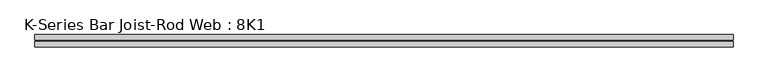
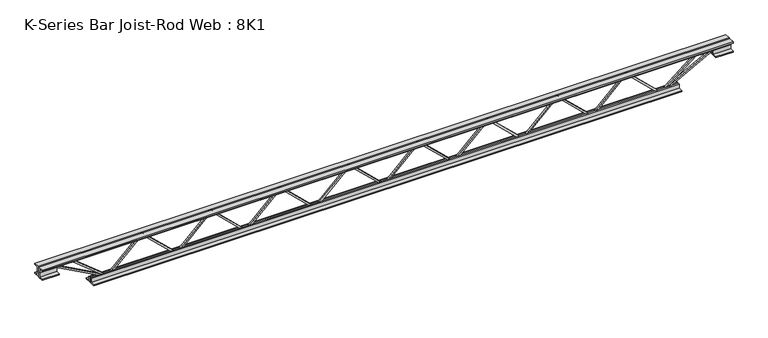
"""IFC4 building model written with IfcOpenShell, lengths in millimetres: beam geometry, K-Series Bar Joist-Rod Web : 8K1."""

from ifc_helpers import new_model, si_unit, frame, origin, place, context, project, spatial, polyline, outline, extrude, source, transform, mapped, element, save


def k_series_bar_joist_rod_web_8k1_28d6b3e6(model_context):
    return source(origin(), model_context, "Body", "SweptSolid", [
        extrude(outline(polyline([(-90.4875, 818.071879), (-100.0125, 818.071879), (-100.0125, 823.1647607), (90.4875, 1021.3327305), (90.4875, 1023.8469671), (-100.0125, 1222.0149368), (-100.0125, 1227.1078185), (-90.4875, 1227.1078185), (-90.4875, 1225.8507002), (100.0125, 1027.6827305), (100.0125, 1017.4969671), (-90.4875, 819.3289973), (-90.4875, 818.071879)])), frame((0.0, -4.7625, 0.0), z_axis=(0.0, 1.0, 0.0), x_axis=(0.0, 0.0, 1.0)), (0.0, 0.0, 1.0), 9.525),
        extrude(outline(polyline([(-90.4875, 409.0359395), (-100.0125, 409.0359395), (-100.0125, 414.1288212), (90.4875, 612.296791), (90.4875, 614.8110276), (-100.0125, 812.9789973), (-100.0125, 818.071879), (-90.4875, 818.071879), (-90.4875, 816.8147607), (100.0125, 618.646791), (100.0125, 608.4610276), (-90.4875, 410.2930578), (-90.4875, 409.0359395)])), frame((0.0, -4.7625, 0.0), z_axis=(0.0, 1.0, 0.0), x_axis=(0.0, 0.0, 1.0)), (0.0, 0.0, 1.0), 9.525),
        extrude(outline(polyline([(-90.4875, 0.0), (-100.0125, 0.0), (-100.0125, 5.0928817), (90.4875, 203.2608514), (90.4875, 205.7750881), (-100.0125, 403.9430578), (-100.0125, 409.0359395), (-90.4875, 409.0359395), (-90.4875, 407.7788212), (100.0125, 209.6108514), (100.0125, 199.4250881), (-90.4875, 1.2571183), (-90.4875, 0.0)])), frame((0.0, -4.7625, 0.0), z_axis=(0.0, 1.0, 0.0), x_axis=(0.0, 0.0, 1.0)), (0.0, 0.0, 1.0), 9.525),
        extrude(outline(polyline([(-90.4875, -409.0359395), (-100.0125, -409.0359395), (-100.0125, -403.9430578), (90.4875, -205.7750881), (90.4875, -203.2608514), (-100.0125, -5.0928817), (-100.0125, 0.0), (-90.4875, 0.0), (-90.4875, -1.2571183), (100.0125, -199.4250881), (100.0125, -209.6108514), (-90.4875, -407.7788212), (-90.4875, -409.0359395)])), frame((0.0, -4.7625, 0.0), z_axis=(0.0, 1.0, 0.0), x_axis=(0.0, 0.0, 1.0)), (0.0, 0.0, 1.0), 9.525),
        extrude(outline(polyline([(-90.4875, -818.071879), (-100.0125, -818.071879), (-100.0125, -812.9789973), (90.4875, -614.8110276), (90.4875, -612.296791), (-100.0125, -414.1288212), (-100.0125, -409.0359395), (-90.4875, -409.0359395), (-90.4875, -410.2930578), (100.0125, -608.4610276), (100.0125, -618.646791), (-90.4875, -816.8147607), (-90.4875, -818.071879)])), frame((0.0, -4.7625, 0.0), z_axis=(0.0, 1.0, 0.0), x_axis=(0.0, 0.0, 1.0)), (0.0, 0.0, 1.0), 9.525),
        extrude(outline(polyline([(-90.4875, -1227.1078185), (-100.0125, -1227.1078185), (-100.0125, -1222.0149368), (90.4875, -1023.8469671), (90.4875, -1021.3327305), (-100.0125, -823.1647607), (-100.0125, -818.071879), (-90.4875, -818.071879), (-90.4875, -819.3289973), (100.0125, -1017.4969671), (100.0125, -1027.6827305), (-90.4875, -1225.8507002), (-90.4875, -1227.1078185)])), frame((0.0, -4.7625, 0.0), z_axis=(0.0, 1.0, 0.0), x_axis=(0.0, 0.0, 1.0)), (0.0, 0.0, 1.0), 9.525),
        extrude(outline(polyline([(-90.4875, 1227.1078185), (-100.0125, 1227.1078185), (-100.0125, 1232.2007002), (90.4875, 1430.36867), (90.4875, 1432.8829066), (-100.0125, 1631.0508764), (-100.0125, 1636.143758), (-90.4875, 1636.143758), (-90.4875, 1634.8866397), (100.0125, 1436.71867), (100.0125, 1426.5329066), (-90.4875, 1228.3649368), (-90.4875, 1227.1078185)])), frame((0.0, -4.7625, 0.0), z_axis=(0.0, 1.0, 0.0), x_axis=(0.0, 0.0, 1.0)), (0.0, 0.0, 1.0), 9.525),
        extrude(outline(polyline([(-90.4875, -1636.143758), (-100.0125, -1636.143758), (-100.0125, -1631.0508764), (90.4875, -1432.8829066), (90.4875, -1430.36867), (-100.0125, -1232.2007002), (-100.0125, -1227.1078185), (-90.4875, -1227.1078185), (-90.4875, -1228.3649368), (100.0125, -1426.5329066), (100.0125, -1436.71867), (-90.4875, -1634.8866397), (-90.4875, -1636.143758)])), frame((0.0, -4.7625, 0.0), z_axis=(0.0, 1.0, 0.0), x_axis=(0.0, 0.0, 1.0)), (0.0, 0.0, 1.0), 9.525),
        extrude(outline(polyline([(4.7625, 101.6), (36.5125, 101.6), (36.5125, 95.25), (11.1125, 95.25), (11.1125, 69.85), (4.7625, 69.85), (4.7625, 101.6)])), frame((-2042.543758, 0.0, 0.0), z_axis=(1.0, 0.0, 0.0), x_axis=(0.0, 1.0, 0.0)), (0.0, 0.0, 1.0), 4085.0875161),
        extrude(outline(polyline([(-4.7625, 101.6), (-4.7625, 69.85), (-11.1125, 69.85), (-11.1125, 95.25), (-36.5125, 95.25), (-36.5125, 101.6), (-4.7625, 101.6)])), frame((-2042.543758, 0.0, 0.0), z_axis=(1.0, 0.0, 0.0), x_axis=(0.0, 1.0, 0.0)), (0.0, 0.0, 1.0), 4085.0875161),
        extrude(outline(polyline([(-4.7625, 38.1), (-36.5125, 38.1), (-36.5125, 44.45), (-11.1125, 44.45), (-11.1125, 69.85), (-4.7625, 69.85), (-4.7625, 38.1)])), frame((-2042.543758, 0.0, 0.0), z_axis=(1.0, 0.0, 0.0), x_axis=(0.0, 1.0, 0.0)), (0.0, 0.0, 1.0), 101.6),
        extrude(outline(polyline([(36.5125, 38.1), (4.7625, 38.1), (4.7625, 69.85), (11.1125, 69.85), (11.1125, 44.45), (36.5125, 44.45), (36.5125, 38.1)])), frame((-2042.543758, 0.0, 0.0), z_axis=(1.0, 0.0, 0.0), x_axis=(0.0, 1.0, 0.0)), (0.0, 0.0, 1.0), 101.6),
        extrude(outline(polyline([(4.7625, 38.1), (4.7625, 69.85), (11.1125, 69.85), (11.1125, 44.45), (36.5125, 44.45), (36.5125, 38.1), (4.7625, 38.1)])), frame((1940.943758, 0.0, 0.0), z_axis=(1.0, 0.0, 0.0), x_axis=(0.0, 1.0, 0.0)), (0.0, 0.0, 1.0), 101.6),
        extrude(outline(polyline([(-4.7625, 38.1), (-36.5125, 38.1), (-36.5125, 44.45), (-11.1125, 44.45), (-11.1125, 69.85), (-4.7625, 69.85), (-4.7625, 38.1)])), frame((1940.943758, 0.0, 0.0), z_axis=(1.0, 0.0, 0.0), x_axis=(0.0, 1.0, 0.0)), (0.0, 0.0, 1.0), 101.6),
        extrude(outline(polyline([(4.7625, -101.6), (4.7625, -69.85), (11.1125, -69.85), (11.1125, -95.25), (36.5125, -95.25), (36.5125, -101.6), (4.7625, -101.6)])), frame((-1737.743758, 0.0, 0.0), z_axis=(1.0, 0.0, 0.0), x_axis=(0.0, 1.0, 0.0)), (0.0, 0.0, 1.0), 3475.4875161),
        extrude(outline(polyline([(-4.7625, -101.6), (-36.5125, -101.6), (-36.5125, -95.25), (-11.1125, -95.25), (-11.1125, -69.85), (-4.7625, -69.85), (-4.7625, -101.6)])), frame((-1737.743758, 0.0, 0.0), z_axis=(1.0, 0.0, 0.0), x_axis=(0.0, 1.0, 0.0)), (0.0, 0.0, 1.0), 3475.4875161),
        extrude(outline(polyline([(0.0, -9.525), (0.0, 0.0), (346.6425392, 0.0), (346.6425392, -9.525), (0.0, -9.525)])), frame((-1943.2120565, 4.7625, 65.662372), z_axis=(0.4762831485400801, 0.0, 0.8792919665371384), x_axis=(0.8792919665371384, 0.0, -0.4762831485400801)), (0.0, 0.0, 1.0), 9.525),
        extrude(outline(polyline([(0.0, -9.525), (0.0, 0.0), (262.841416, 0.0), (262.841416, -9.525), (0.0, -9.525)])), frame((-1843.6532227, 4.7625, 66.1442795), z_axis=(0.6281354077548245, 0.0, 0.7781040480068719), x_axis=(0.7781040480068719, 0.0, -0.6281354077548245)), (0.0, 0.0, 1.0), 9.525),
        extrude(outline(polyline([(0.0, -9.525), (0.0, 0.0), (346.6425392, 0.0), (346.6425392, -9.525), (0.0, -9.525)])), frame((1943.2120565, -4.7625, 65.662372), z_axis=(-0.47628314854004167, 0.0, 0.8792919665371591), x_axis=(-0.8792919665371591, 0.0, -0.47628314854004167)), (0.0, 0.0, 1.0), 9.525),
        extrude(outline(polyline([(0.0, -9.525), (0.0, 0.0), (262.841416, 0.0), (262.841416, -9.525), (0.0, -9.525)])), frame((1843.6532227, -4.7625, 66.1442795), z_axis=(-0.6281354077547995, 0.0, 0.778104048006892), x_axis=(-0.778104048006892, 0.0, -0.6281354077547995)), (0.0, 0.0, 1.0), 9.525),
    ])


if __name__ == "__main__":
    model = new_model("IFC4")
    model_context = context("Model", 3, world=origin())
    ifc_project = project(units=[si_unit("LENGTHUNIT", "METRE", prefix="MILLI")], contexts=[model_context])
    site = spatial("IfcSite", under=ifc_project)
    building = spatial("IfcBuilding", under=site)
    placement = place(None, origin())
    k_series_bar_joist_rod_web_8k1_shape = k_series_bar_joist_rod_web_8k1_28d6b3e6(model_context)
    element("IfcBeam", 1, ObjectType="K-Series Bar Joist-Rod Web : 8K1", at=placement, inside=building, context=model_context, shape_type="MappedRepresentation", body=[
        mapped(k_series_bar_joist_rod_web_8k1_shape, transform((0.0, 0.0, 0.0), x_axis=(1.0, 0.0, 0.0), y_axis=(0.0, 1.0, 0.0), z_axis=(0.0, 0.0, 1.0))),
    ])
    save(model, "model.ifc")

# Revit data of these elements
# Type "K-Series Bar Joist-Rod Web : 8K1"
#   Assembly Code = "B1010350"
#   Wt = 5.1
#   Web Thickness = 0' - 0 3/8"
#   Start Offset [instance default] = 0' - 0"
#   Start Extension [instance default] = 0' - 0"
#   Seat Length = 0' - 4"
#   Seat Depth = 0' - 2 1/2"
#   PanelArrayLength [instance default] = 21' - 4"
#   Panel [instance default] = 1' - 4"
#   End Offset [instance default] = 0' - 0"
#   End Extension [instance default] = 0' - 0"
#   End Panel = 1' - 4"
#   Cord Leg = 0' - 1 1/4"
#   Chord Thickness = 0' - 0 1/4"
#   Length [instance default] = 24' - 0"
#   Depth = 0' - 8"
#   PanelArrayNum [instance default] = 16
#   Rendering Material = none
# Element 1 (IfcBeam, "K-Series Bar Joist-Rod Web : 8K1")
#   PanelArrayLength = 10' - 8.83022"
#   Panel = 1' - 4.10378"
#   PanelArrayNum = 8
